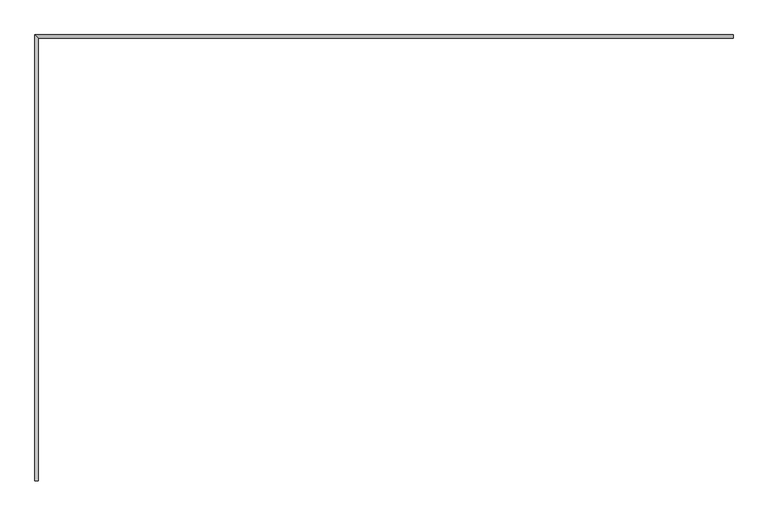
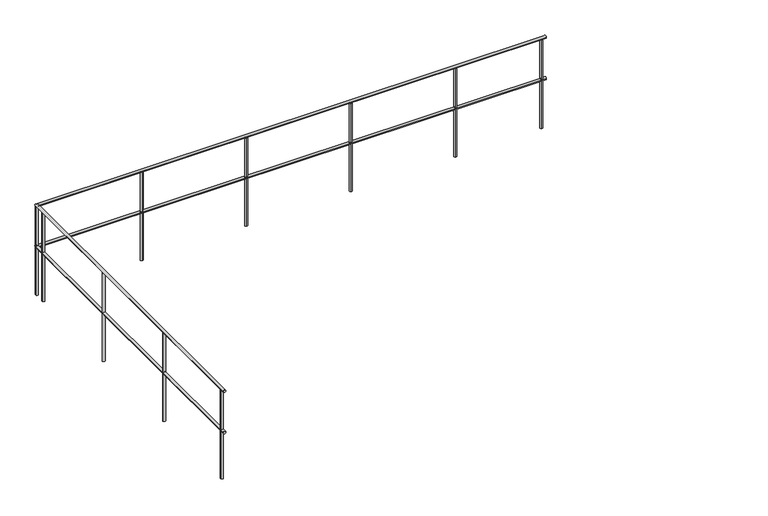
"""IFC4 building model written with IfcOpenShell, lengths in millimetres: railing geometry."""

from ifc_helpers import new_model, si_unit, point, frame, frame_2d, origin, place, context, project, spatial, circle_curve, ellipse_curve, trimmed, segment, composite_curve, outline, extrude, source, transform, mapped, element, save
from ifc_brep_helpers import plane_surface, cylinder_surface, advanced_brep


def railing_5d0c8113(model_context):
    return source(origin(), model_context, "Body", "SolidModel", [
        advanced_brep(
        [(25710.0, 60949.5208589, 885.0), (25740.0, 60949.5208589, 885.0), (25710.0, 64692.0208589, 885.0), (25740.0, 64662.0208589, 885.0), (31562.1378478, 64692.0208589, 885.0), (31562.1378478, 64662.0208589, 885.0)],
        [
            (0, 1, circle_curve(frame((25725.0, 60949.5208589, 885.0), z_axis=(0.0, -1.0, 0.0), x_axis=(1.0, 0.0, 0.0)), 15.0)),
            (1, 0, circle_curve(frame((25725.0, 60949.5208589, 885.0), z_axis=(0.0, -1.0, 0.0), x_axis=(1.0, 0.0, 0.0)), 15.0)),
            (0, 2),
            (2, 3, ellipse_curve(frame((25725.0, 64677.0208589, 885.0), z_axis=(-0.7071067811865489, -0.7071067811865461, 0.0), x_axis=(0.707106781186546, -0.7071067811865489, 0.0)), 21.2132034, 15.0)),
            (3, 1),
            (3, 2, ellipse_curve(frame((25725.0, 64677.0208589, 885.0), z_axis=(-0.7071067811865489, -0.7071067811865461, 0.0), x_axis=(0.707106781186546, -0.7071067811865489, 0.0)), 21.2132034, 15.0)),
            (4, 5, circle_curve(frame((31562.1378478, 64677.0208589, 885.0), z_axis=(1.0, 0.0, 0.0), x_axis=(0.0, -1.0, 0.0)), 15.0)),
            (5, 4, circle_curve(frame((31562.1378478, 64677.0208589, 885.0), z_axis=(1.0, 0.0, 0.0), x_axis=(0.0, -1.0, 0.0)), 15.0)),
            (2, 4),
            (5, 3),
        ],
        [
            plane_surface(frame((25725.0, 60949.5208589, 900.0), z_axis=(0.0, -1.0, 0.0), x_axis=(0.0, 0.0, 1.0))),
            cylinder_surface(frame((25725.0, 60949.5208589, 885.0), z_axis=(0.0, -1.0, 0.0), x_axis=(1.0, 0.0, 0.0)), 15.0),
            plane_surface(frame((31562.1378478, 64677.0208589, 900.0), z_axis=(1.0, 0.0, 0.0), x_axis=(0.0, 1.0, 0.0))),
            cylinder_surface(frame((25725.0, 64677.0208589, 885.0), z_axis=(-1.0, 0.0, 0.0), x_axis=(0.0, -1.0, 0.0)), 15.0),
        ],
        [
            (0, [[1, 2]]),
            (1, [[-1, 3, 4, 5]]),
            (1, [[-2, -5, 6, -3]]),
            (2, [[7, 8]]),
            (3, [[-4, 9, -8, 10]]),
            (3, [[-6, -10, -7, -9]]),
        ],
    ),
        advanced_brep(
        [(25710.0, 60949.5208589, 1385.0), (25740.0, 60949.5208589, 1385.0), (25710.0, 64692.0208589, 1385.0), (25740.0, 64662.0208589, 1385.0), (31562.1378478, 64692.0208589, 1385.0), (31562.1378478, 64662.0208589, 1385.0)],
        [
            (0, 1, circle_curve(frame((25725.0, 60949.5208589, 1385.0), z_axis=(0.0, -1.0, 0.0), x_axis=(1.0, 0.0, 0.0)), 15.0)),
            (1, 0, circle_curve(frame((25725.0, 60949.5208589, 1385.0), z_axis=(0.0, -1.0, 0.0), x_axis=(1.0, 0.0, 0.0)), 15.0)),
            (0, 2),
            (2, 3, ellipse_curve(frame((25725.0, 64677.0208589, 1385.0), z_axis=(-0.7071067811865489, -0.7071067811865461, 0.0), x_axis=(0.707106781186546, -0.7071067811865489, 0.0)), 21.2132034, 15.0)),
            (3, 1),
            (3, 2, ellipse_curve(frame((25725.0, 64677.0208589, 1385.0), z_axis=(-0.7071067811865489, -0.7071067811865461, 0.0), x_axis=(0.707106781186546, -0.7071067811865489, 0.0)), 21.2132034, 15.0)),
            (4, 5, circle_curve(frame((31562.1378478, 64677.0208589, 1385.0), z_axis=(1.0, 0.0, 0.0), x_axis=(0.0, -1.0, 0.0)), 15.0)),
            (5, 4, circle_curve(frame((31562.1378478, 64677.0208589, 1385.0), z_axis=(1.0, 0.0, 0.0), x_axis=(0.0, -1.0, 0.0)), 15.0)),
            (2, 4),
            (5, 3),
        ],
        [
            plane_surface(frame((25725.0, 60949.5208589, 1400.0), z_axis=(0.0, -1.0, 0.0), x_axis=(0.0, 0.0, 1.0))),
            cylinder_surface(frame((25725.0, 60949.5208589, 1385.0), z_axis=(0.0, -1.0, 0.0), x_axis=(1.0, 0.0, 0.0)), 15.0),
            plane_surface(frame((31562.1378478, 64677.0208589, 1400.0), z_axis=(1.0, 0.0, 0.0), x_axis=(0.0, 1.0, 0.0))),
            cylinder_surface(frame((25725.0, 64677.0208589, 1385.0), z_axis=(-1.0, 0.0, 0.0), x_axis=(0.0, -1.0, 0.0)), 15.0),
        ],
        [
            (0, [[1, 2]]),
            (1, [[-1, 3, 4, 5]]),
            (1, [[-2, -5, 6, -3]]),
            (2, [[7, 8]]),
            (3, [[-4, 9, -8, 10]]),
            (3, [[-6, -10, -7, -9]]),
        ],
    ),
        extrude(outline(composite_curve([segment(trimmed(circle_curve(frame_2d((30525.0, 64677.0208589)), 15.0), [point((30525.0, 64692.0208589))], [point((30525.0, 64662.0208589))], False, "CARTESIAN"), True, "CONTINUOUS"), segment(trimmed(circle_curve(frame_2d((30525.0, 64677.0208589)), 15.0), [point((30525.0, 64662.0208589))], [point((30525.0, 64692.0208589))], False, "CARTESIAN"), True, "CONTINUOUS")], self_intersect=False)), frame((0.0, 0.0, 300.0), z_axis=(0.0, 0.0, 1.0), x_axis=(1.0, 0.0, 0.0)), (0.0, 0.0, 1.0), 1070.0),
        extrude(outline(composite_curve([segment(trimmed(circle_curve(frame_2d((29325.0, 64677.0208589)), 15.0), [point((29325.0, 64692.0208589))], [point((29325.0, 64662.0208589))], False, "CARTESIAN"), True, "CONTINUOUS"), segment(trimmed(circle_curve(frame_2d((29325.0, 64677.0208589)), 15.0), [point((29325.0, 64662.0208589))], [point((29325.0, 64692.0208589))], False, "CARTESIAN"), True, "CONTINUOUS")], self_intersect=False)), frame((0.0, 0.0, 300.0), z_axis=(0.0, 0.0, 1.0), x_axis=(1.0, 0.0, 0.0)), (0.0, 0.0, 1.0), 1070.0),
        extrude(outline(composite_curve([segment(trimmed(circle_curve(frame_2d((28125.0, 64677.0208589)), 15.0), [point((28125.0, 64692.0208589))], [point((28125.0, 64662.0208589))], False, "CARTESIAN"), True, "CONTINUOUS"), segment(trimmed(circle_curve(frame_2d((28125.0, 64677.0208589)), 15.0), [point((28125.0, 64662.0208589))], [point((28125.0, 64692.0208589))], False, "CARTESIAN"), True, "CONTINUOUS")], self_intersect=False)), frame((0.0, 0.0, 300.0), z_axis=(0.0, 0.0, 1.0), x_axis=(1.0, 0.0, 0.0)), (0.0, 0.0, 1.0), 1070.0),
        extrude(outline(composite_curve([segment(trimmed(circle_curve(frame_2d((26925.0, 64677.0208589)), 15.0), [point((26925.0, 64692.0208589))], [point((26925.0, 64662.0208589))], False, "CARTESIAN"), True, "CONTINUOUS"), segment(trimmed(circle_curve(frame_2d((26925.0, 64677.0208589)), 15.0), [point((26925.0, 64662.0208589))], [point((26925.0, 64692.0208589))], False, "CARTESIAN"), True, "CONTINUOUS")], self_intersect=False)), frame((0.0, 0.0, 300.0), z_axis=(0.0, 0.0, 1.0), x_axis=(1.0, 0.0, 0.0)), (0.0, 0.0, 1.0), 1070.0),
        extrude(outline(composite_curve([segment(trimmed(circle_curve(frame_2d((25725.0, 64549.5208589)), 15.0), [point((25710.0, 64549.5208589))], [point((25740.0, 64549.5208589))], False, "CARTESIAN"), True, "CONTINUOUS"), segment(trimmed(circle_curve(frame_2d((25725.0, 64549.5208589)), 15.0), [point((25740.0, 64549.5208589))], [point((25710.0, 64549.5208589))], False, "CARTESIAN"), True, "CONTINUOUS")], self_intersect=False)), frame((0.0, 0.0, 300.0), z_axis=(0.0, 0.0, 1.0), x_axis=(1.0, 0.0, 0.0)), (0.0, 0.0, 1.0), 1070.0),
        extrude(outline(composite_curve([segment(trimmed(circle_curve(frame_2d((25725.0, 63349.5208589)), 15.0), [point((25710.0, 63349.5208589))], [point((25740.0, 63349.5208589))], False, "CARTESIAN"), True, "CONTINUOUS"), segment(trimmed(circle_curve(frame_2d((25725.0, 63349.5208589)), 15.0), [point((25740.0, 63349.5208589))], [point((25710.0, 63349.5208589))], False, "CARTESIAN"), True, "CONTINUOUS")], self_intersect=False)), frame((0.0, 0.0, 300.0), z_axis=(0.0, 0.0, 1.0), x_axis=(1.0, 0.0, 0.0)), (0.0, 0.0, 1.0), 1070.0),
        extrude(outline(composite_curve([segment(trimmed(circle_curve(frame_2d((25725.0, 62149.5208589)), 15.0), [point((25710.0, 62149.5208589))], [point((25740.0, 62149.5208589))], False, "CARTESIAN"), True, "CONTINUOUS"), segment(trimmed(circle_curve(frame_2d((25725.0, 62149.5208589)), 15.0), [point((25740.0, 62149.5208589))], [point((25710.0, 62149.5208589))], False, "CARTESIAN"), True, "CONTINUOUS")], self_intersect=False)), frame((0.0, 0.0, 300.0), z_axis=(0.0, 0.0, 1.0), x_axis=(1.0, 0.0, 0.0)), (0.0, 0.0, 1.0), 1070.0),
        extrude(outline(composite_curve([segment(trimmed(circle_curve(frame_2d((25725.0, 64677.0208589)), 15.0), [point((25710.0, 64677.0208589))], [point((25740.0, 64677.0208589))], False, "CARTESIAN"), True, "CONTINUOUS"), segment(trimmed(circle_curve(frame_2d((25725.0, 64677.0208589)), 15.0), [point((25740.0, 64677.0208589))], [point((25710.0, 64677.0208589))], False, "CARTESIAN"), True, "CONTINUOUS")], self_intersect=False)), frame((0.0, 0.0, 300.0), z_axis=(0.0, 0.0, 1.0), x_axis=(1.0, 0.0, 0.0)), (0.0, 0.0, 1.0), 1070.0),
        extrude(outline(composite_curve([segment(trimmed(circle_curve(frame_2d((31512.1378478, 64677.0208589)), 15.0), [point((31512.1378478, 64692.0208589))], [point((31512.1378478, 64662.0208589))], False, "CARTESIAN"), True, "CONTINUOUS"), segment(trimmed(circle_curve(frame_2d((31512.1378478, 64677.0208589)), 15.0), [point((31512.1378478, 64662.0208589))], [point((31512.1378478, 64692.0208589))], False, "CARTESIAN"), True, "CONTINUOUS")], self_intersect=False)), frame((0.0, 0.0, 300.0), z_axis=(0.0, 0.0, 1.0), x_axis=(1.0, 0.0, 0.0)), (0.0, 0.0, 1.0), 1070.0),
        extrude(outline(composite_curve([segment(trimmed(circle_curve(frame_2d((25725.0, 60999.5208589)), 15.0), [point((25710.0, 60999.5208589))], [point((25740.0, 60999.5208589))], False, "CARTESIAN"), True, "CONTINUOUS"), segment(trimmed(circle_curve(frame_2d((25725.0, 60999.5208589)), 15.0), [point((25740.0, 60999.5208589))], [point((25710.0, 60999.5208589))], False, "CARTESIAN"), True, "CONTINUOUS")], self_intersect=False)), frame((0.0, 0.0, 300.0), z_axis=(0.0, 0.0, 1.0), x_axis=(1.0, 0.0, 0.0)), (0.0, 0.0, 1.0), 1070.0),
    ])


if __name__ == "__main__":
    model = new_model("IFC4")
    model_context = context("Model", 3, world=origin())
    ifc_project = project(units=[si_unit("LENGTHUNIT", "METRE", prefix="MILLI")], contexts=[model_context])
    site = spatial("IfcSite", under=ifc_project)
    building = spatial("IfcBuilding", under=site)
    placement = place(None, origin())
    railing_shape = railing_5d0c8113(model_context)
    element("IfcRailing", 1, at=placement, inside=building, context=model_context, shape_type="MappedRepresentation", body=[
        mapped(railing_shape, transform((0.0, 0.0, 0.0), x_axis=(1.0, 0.0, 0.0), y_axis=(0.0, 1.0, 0.0), z_axis=(0.0, 0.0, 1.0))),
    ])
    save(model, "model.ifc")
